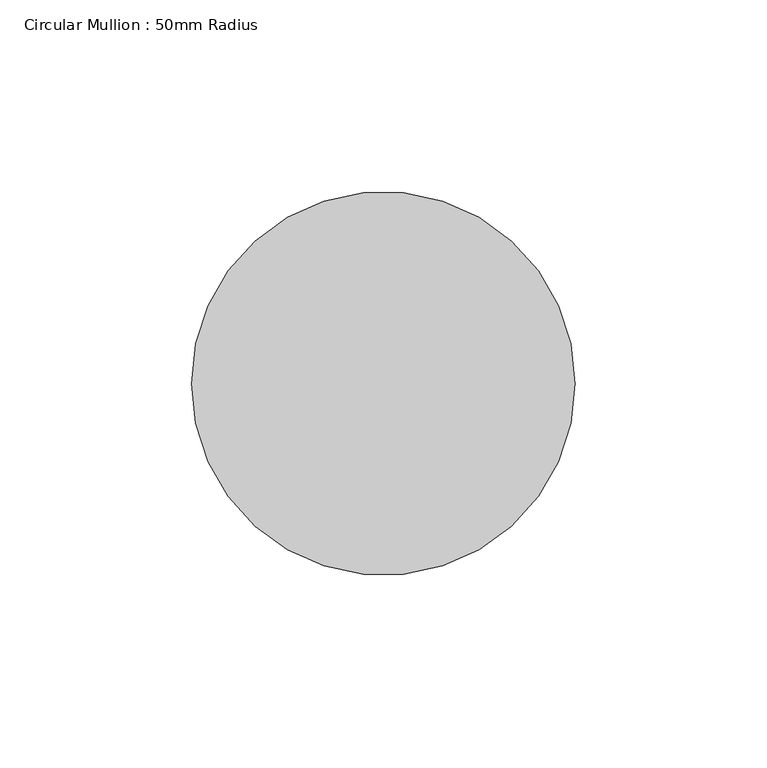
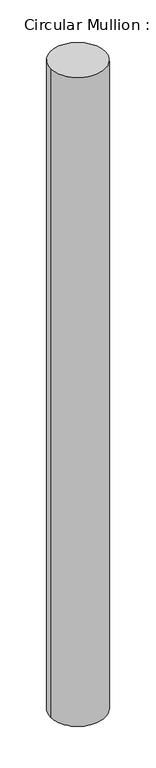
"""IFC4 building model written with IfcOpenShell, lengths in millimetres: member geometry, Circular Mullion : 50mm Radius."""

from ifc_helpers import new_model, si_unit, frame, origin, place, context, project, spatial, ellipse_curve, source, transform, mapped, element, save
from ifc_brep_helpers import plane_surface, cylinder_surface, advanced_brep


def circular_mullion_50mm_radius_12e1bb08(model_context):
    return source(origin(), model_context, "Body", "AdvancedBrep", [
        advanced_brep(
        [(-100.0, 0.0, 0.716886), (0.0, 0.0, 0.0), (0.0, 0.0, -1251.858137), (-100.0, 0.0, -1252.6211973)],
        [
            (0, 1, ellipse_curve(frame((-50.0, 0.0, 0.358443), z_axis=(-0.007167581643917269, -0.01746971925426822, -0.9998217014460903), x_axis=(-0.37951212764758363, -0.9249940430353912, 0.018882937203862984)), 50.0089165, 50.0)),
            (1, 2),
            (2, 3, ellipse_curve(frame((-50.0, 0.0, -1252.2396671), z_axis=(-0.007629061269405463, -0.018594494652631608, 0.9997980006945208), x_axis=(0.3795031313209074, 0.9249721160718236, 0.020098701630670235)), 50.010102, 50.0)),
            (3, 0),
            (1, 0, ellipse_curve(frame((-50.0, 0.0, 0.358443), z_axis=(-0.007167581643917269, -0.01746971925426822, -0.9998217014460903), x_axis=(-0.37951212764758363, -0.9249940430353912, 0.018882937203862984)), 50.0089165, 50.0)),
            (3, 2, ellipse_curve(frame((-50.0, 0.0, -1252.2396671), z_axis=(-0.007629061269405463, -0.018594494652631608, 0.9997980006945208), x_axis=(0.3795031313209074, 0.9249721160718236, 0.020098701630670235)), 50.010102, 50.0)),
        ],
        [
            cylinder_surface(frame((-50.0, 0.0, 0.0), z_axis=(0.0, 0.0, 1.0), x_axis=(1.0, 0.0, 0.0)), 50.0),
            plane_surface(frame((-281.9884625, 115.6959249, 0.0), z_axis=(0.00716758164391727, 0.017469719254268223, 0.9998217014460905), x_axis=(0.37951212764758346, 0.9249940430353912, -0.018882937203866603))),
            plane_surface(frame((-281.9884625, 115.6959249, -1251.858137), z_axis=(0.007629061269405463, 0.018594494652631608, -0.9997980006945208), x_axis=(0.37950313132090735, 0.9249721160718236, 0.020098701630679727))),
        ],
        [
            (0, [[1, 2, 3, 4]]),
            (0, [[5, -4, 6, -2]]),
            (1, [[-1, -5]]),
            (2, [[-6, -3]]),
        ],
    ),
    ])


if __name__ == "__main__":
    model = new_model("IFC4")
    model_context = context("Model", 3, world=origin())
    ifc_project = project(units=[si_unit("LENGTHUNIT", "METRE", prefix="MILLI")], contexts=[model_context])
    site = spatial("IfcSite", under=ifc_project)
    building = spatial("IfcBuilding", under=site)
    placement = place(None, origin())
    circular_mullion_50mm_radius_shape = circular_mullion_50mm_radius_12e1bb08(model_context)
    element("IfcMember", 1, ObjectType="Circular Mullion : 50mm Radius", at=placement, inside=building, context=model_context, shape_type="MappedRepresentation", body=[
        mapped(circular_mullion_50mm_radius_shape, transform((0.0, 0.0, 0.0), x_axis=(1.0, 0.0, 0.0), y_axis=(0.0, 1.0, 0.0), z_axis=(0.0, 0.0, 1.0))),
    ])
    save(model, "model.ifc")

# Revit data of these elements
# Type "Circular Mullion : 50mm Radius"
#   built-in parameter 1007350 = 0.164042 (stored number, unit not read)
# Element 1 (IfcMember, "Circular Mullion : 50mm Radius")
#   Materials on its faces: "Aluminium"
# Materials
#   "Aluminium": class "Metal", colour RGB 247 247 247, transparency 0, Description = "Aluminium 6061", Cost = 0
